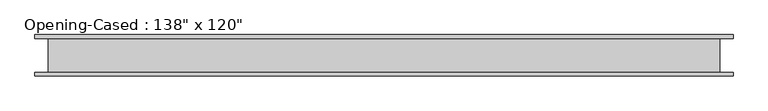
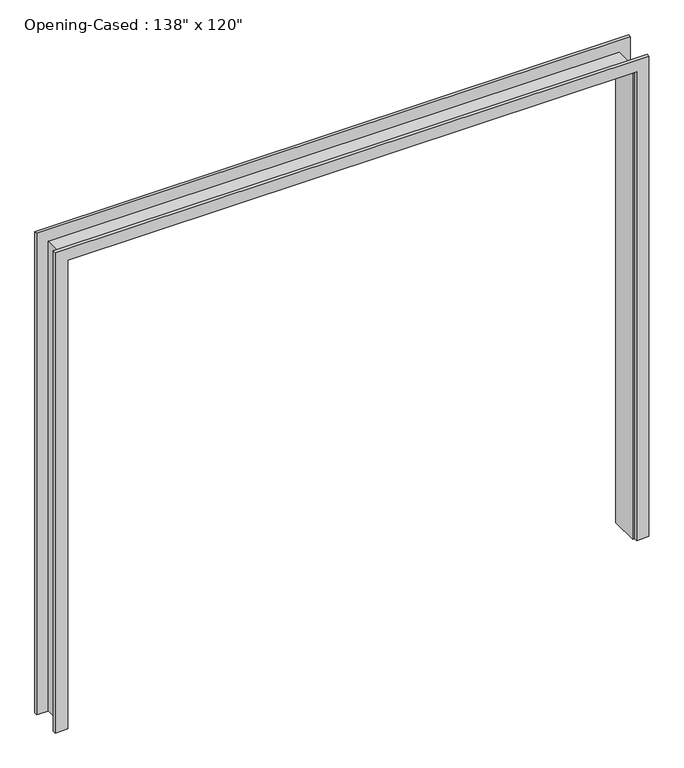
"""IFC4 building model written with IfcOpenShell, lengths in millimetres: proxy geometry."""

from ifc_helpers import new_model, si_unit, frame, origin, place, context, project, spatial, polyline, outline, extrude, faceted_brep, source, transform, mapped, element, save


def proxy_bf856442(model_context):
    return source(origin(), model_context, "Body", "SolidModel", [
        extrude(outline(polyline([(0.0, -1754.4386567), (3041.65, -1754.4386567), (3041.65, 1738.0613433), (0.0, 1738.0613433), (0.0, 1814.2613433), (3117.85, 1814.2613433), (3117.85, -1830.6386567), (0.0, -1830.6386567), (0.0, -1754.4386567)])), frame((0.0, -107.95, 0.0), z_axis=(0.0, 1.0, 0.0), x_axis=(0.0, 0.0, 1.0)), (0.0, 0.0, 1.0), 19.05),
        extrude(outline(polyline([(0.0, 1814.2613433), (3124.2, 1814.2613433), (3124.2, -1830.6386567), (0.0, -1830.6386567), (0.0, -1754.4386567), (3041.65, -1754.4386567), (3041.65, 1738.0613433), (0.0, 1738.0613433), (0.0, 1814.2613433)])), frame((0.0, 88.9, 0.0), z_axis=(0.0, 1.0, 0.0), x_axis=(0.0, 0.0, 1.0)), (0.0, 0.0, 1.0), 19.05),
        faceted_brep([(1725.3613433, 88.9, 0.0), (1744.4113433, 88.9, 0.0), (1744.4113433, -88.9, 0.0), (1725.3613433, -88.9, 0.0), (1725.3613433, 88.9, 3028.95), (1744.4113433, 88.9, 3048.0), (1744.4113433, -88.9, 3048.0), (1725.3613433, -88.9, 3028.95), (-1741.7386567, 88.9, 3028.95), (-1760.7886567, 88.9, 3048.0), (-1760.7886567, -88.9, 3048.0), (-1741.7386567, -88.9, 3028.95), (-1741.7386567, 88.9, 0.0), (-1741.7386567, -88.9, 0.0), (-1760.7886567, -88.9, 0.0), (-1760.7886567, 88.9, 0.0)], [[[0, 1, 2, 3]], [[1, 0, 4, 5]], [[2, 1, 5, 6]], [[3, 2, 6, 7]], [[0, 3, 7, 4]], [[5, 4, 8, 9]], [[6, 5, 9, 10]], [[7, 6, 10, 11]], [[4, 7, 11, 8]], [[12, 13, 14, 15]], [[9, 8, 12, 15]], [[10, 9, 15, 14]], [[11, 10, 14, 13]], [[8, 11, 13, 12]]]),
    ])


if __name__ == "__main__":
    model = new_model("IFC4")
    model_context = context("Model", 3, world=origin())
    ifc_project = project(units=[si_unit("LENGTHUNIT", "METRE", prefix="MILLI")], contexts=[model_context])
    site = spatial("IfcSite", under=ifc_project)
    building = spatial("IfcBuilding", under=site)
    placement = place(None, origin())
    proxy_shape = proxy_bf856442(model_context)
    element("IfcBuildingElementProxy", 1, Name="Opening-Cased : 138\" x 120\"", ObjectType="Opening-Cased : 138\" x 120\"", at=placement, inside=building, context=model_context, shape_type="MappedRepresentation", body=[
        mapped(proxy_shape, transform((0.0, 0.0, 0.0), x_axis=(1.0, 0.0, 0.0), y_axis=(0.0, 1.0, 0.0), z_axis=(0.0, 0.0, 1.0))),
    ])
    save(model, "model.ifc")

# Revit data of these elements
# Type "Opening-Cased : 138\" x 120\""
#   Height = 3048 mm
#   Trim Thickness = 19.05 mm
#   Trim Width = 76.2 mm
#   Width = 3505.2 mm
#   Frame Material = Door - Frame
#   Default Elevation = 0
# Element 1 (IfcBuildingElementProxy, "Opening-Cased : 138\" x 120\"")
#   Materials on its faces: "Door - Frame"
# Materials
#   "Door - Frame": class "Miscellaneous", colour RGB 118 70 51, transparency 0
